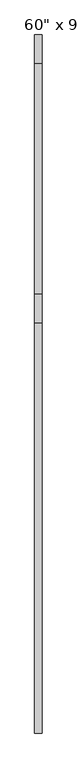
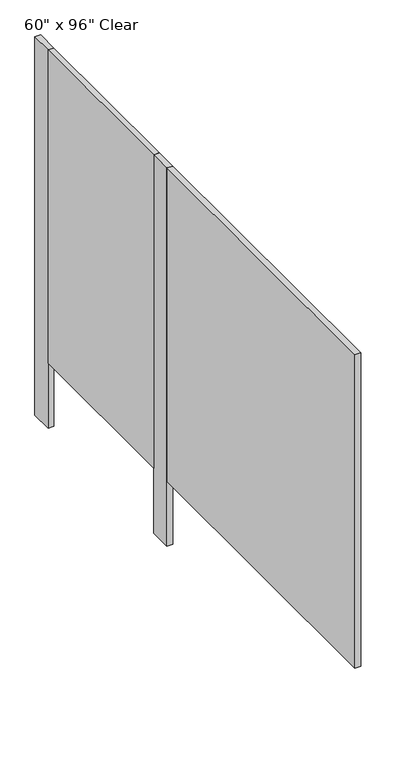
"""IFC4 building model written with IfcOpenShell, lengths in millimetres: proxy geometry."""

import ifcopenshell
import ifcopenshell.guid

model = None  # the IFC model being written
_history = None  # IfcOwnerHistory: only IFC2X3 demands one
_inside = {}  # id of a spatial element -> (the spatial element, [elements in it])
_under = {}  # id of a project, library or spatial element -> (it, [spatial elements below it])
_declared = {}  # id of a project -> (the project, [libraries it declares])
_typed = {}  # id of a type object -> (the type object, [elements of that type])
_made_of = {}  # id of a material, layer set ... -> (it, [elements and type objects made of it])


def new_model(schema):
    """Start an empty IFC model of exactly this schema.

    Asked for "IFC4X3", IfcOpenShell would pick the latest addendum, in which some entities
    have other attributes; the version numbers below select the first issue.
    IFC2X3 requires an IfcOwnerHistory on every rooted entity: one is made here for all.
    """
    global model, _history
    if schema == "IFC4X3":
        model = ifcopenshell.file(schema_version=(4, 3, 0, 0))
    else:
        model = ifcopenshell.file(schema=schema)
    _inside.clear()
    _under.clear()
    _declared.clear()
    _typed.clear()
    _made_of.clear()
    _history = None
    if model.schema == "IFC2X3":
        org = make("IfcOrganization", Name="unknown")
        user = make(
            "IfcPersonAndOrganization",
            ThePerson=make("IfcPerson", FamilyName="unknown"),
            TheOrganization=org,
        )
        app = make(
            "IfcApplication",
            ApplicationDeveloper=org,
            Version="unknown",
            ApplicationFullName="unknown",
            ApplicationIdentifier="unknown",
        )
        _history = make(
            "IfcOwnerHistory",
            OwningUser=user,
            OwningApplication=app,
            ChangeAction="ADDED",
            CreationDate=0,
        )
    return model


def make(cls, **values):
    """One entity of the class cls with the attributes given. An attribute that is None is left unset."""
    return model.create_entity(
        cls, **{name: value for name, value in values.items() if value is not None}
    )


def rooted(cls, **values):
    """An entity with a GlobalId (a new one), such as an element, a storey or a relation."""
    return make(cls, GlobalId=ifcopenshell.guid.new(), OwnerHistory=_history, **values)


def si_unit(unit_type, name, prefix=None):
    """IfcSIUnit, for example si_unit("LENGTHUNIT", "METRE", prefix="MILLI")."""
    return make("IfcSIUnit", UnitType=unit_type, Prefix=prefix, Name=name)


def assignment(units):
    """IfcUnitAssignment: the units of a project."""
    return None if units is None else make("IfcUnitAssignment", Units=units)


def point(xyz):
    """IfcCartesianPoint."""
    return None if xyz is None else make("IfcCartesianPoint", Coordinates=xyz)


def direction(xyz):
    """IfcDirection."""
    return None if xyz is None else make("IfcDirection", DirectionRatios=xyz)


def frame(location, z_axis=None, x_axis=None):
    """IfcAxis2Placement3D, a coordinate frame: its origin and axes. An axis left out is left unset."""
    return make(
        "IfcAxis2Placement3D",
        Location=point(location),
        Axis=direction(z_axis),
        RefDirection=direction(x_axis),
    )


def origin():
    """The frame at (0, 0, 0) with its axes left unset."""
    return frame((0.0, 0.0, 0.0))


def origin_with_axes():
    """The frame at (0, 0, 0) with the z axis (0, 0, 1) and the x axis (1, 0, 0) written out."""
    return frame((0.0, 0.0, 0.0), z_axis=(0.0, 0.0, 1.0), x_axis=(1.0, 0.0, 0.0))


def place(relative_to, where):
    """IfcLocalPlacement: puts the frame where relative to a parent placement (None: the world)."""
    return make(
        "IfcLocalPlacement", PlacementRelTo=relative_to, RelativePlacement=where
    )


def context(
    kind, dimensions, precision=None, world=None, true_north=None, identifier=None
):
    """IfcGeometricRepresentationContext, for example the 3D "Model" context."""
    return make(
        "IfcGeometricRepresentationContext",
        ContextIdentifier=identifier,
        ContextType=kind,
        CoordinateSpaceDimension=dimensions,
        Precision=precision,
        WorldCoordinateSystem=world,
        TrueNorth=true_north,
    )


def project(units=None, contexts=None):
    """IfcProject with its units and contexts."""
    return rooted(
        "IfcProject",
        Name="project",
        RepresentationContexts=contexts,
        UnitsInContext=assignment(units),
    )


def spatial(cls, under=None, at=None, **own):
    """A site, building, storey or space (cls), placed at a placement, below another one or the project."""
    s = rooted(cls, ObjectPlacement=at, **own)
    if under is not None:
        _under.setdefault(under.id(), (under, []))[1].append(s)
    return s


def polyline(points):
    """IfcPolyline through the points."""
    return make("IfcPolyline", Points=[point(p) for p in points])


def outline(outer, holes=None, kind="AREA"):
    """IfcArbitraryClosedProfileDef: a profile drawn as a closed curve; with holes, ...WithVoids."""
    if holes is None:
        return make("IfcArbitraryClosedProfileDef", ProfileType=kind, OuterCurve=outer)
    return make(
        "IfcArbitraryProfileDefWithVoids",
        ProfileType=kind,
        OuterCurve=outer,
        InnerCurves=holes,
    )


def extrude(swept, where, along, depth):
    """IfcExtrudedAreaSolid: the profile swept, set in the frame where, extruded along a direction by depth."""
    return make(
        "IfcExtrudedAreaSolid",
        SweptArea=swept,
        Position=where,
        ExtrudedDirection=direction(along),
        Depth=depth,
    )


def shape(context_of_items, identifier, shape_type, items):
    """IfcShapeRepresentation: the items that make up one representation, for example the "Body"."""
    return make(
        "IfcShapeRepresentation",
        ContextOfItems=context_of_items,
        RepresentationIdentifier=identifier,
        RepresentationType=shape_type,
        Items=items,
    )


def source(mapping_origin, context_of_items, identifier, shape_type, items):
    """IfcRepresentationMap: a shape defined once, which mapped items show again and again."""
    return make(
        "IfcRepresentationMap",
        MappingOrigin=mapping_origin,
        MappedRepresentation=shape(context_of_items, identifier, shape_type, items),
    )


def transform(
    local_origin,
    x_axis=None,
    y_axis=None,
    z_axis=None,
    scale=None,
    scale2=None,
    scale3=None,
    uniform=True,
):
    """IfcCartesianTransformationOperator3D, or its non-uniform kind. x_axis, y_axis, z_axis: its Axis1, 2, 3."""
    if uniform:
        return make(
            "IfcCartesianTransformationOperator3D",
            Axis1=direction(x_axis),
            Axis2=direction(y_axis),
            LocalOrigin=point(local_origin),
            Scale=scale,
            Axis3=direction(z_axis),
        )
    return make(
        "IfcCartesianTransformationOperator3DnonUniform",
        Axis1=direction(x_axis),
        Axis2=direction(y_axis),
        LocalOrigin=point(local_origin),
        Scale=scale,
        Axis3=direction(z_axis),
        Scale2=scale2,
        Scale3=scale3,
    )


def mapped(mapping_source, mapping_target):
    """IfcMappedItem: shows the shape of a source again, moved by a transform."""
    return make(
        "IfcMappedItem", MappingSource=mapping_source, MappingTarget=mapping_target
    )


def made_of(thing, what):
    """Note that an element or type object is made of a material, layer set ...; save() writes the relation."""
    if what is not None:
        _made_of.setdefault(what.id(), (what, []))[1].append(thing)
    return thing


def element(
    cls,
    number,
    at=None,
    inside=None,
    cuts=None,
    type_object=None,
    material=None,
    context=None,
    identifier="Body",
    shape_type=None,
    held_by="IfcProductDefinitionShape",
    body=None,
    shapes=None,
    **own,
):
    """One element of the class cls, such as IfcWall. Its Tag is "e" and its number.

    at: its placement. inside: the storey or other place that contains it. cuts: it is an
    opening in that element (IfcRelVoidsElement). A single representation is given by context,
    identifier, shape_type and body (its items); several are given by shapes. held_by: the class
    of the entity that holds the representations. save() writes the other relations.
    """
    e = rooted(cls, Tag="e%d" % number, ObjectPlacement=at, **own)
    if body is not None:
        shapes = [shape(context, identifier, shape_type, body)]
    if shapes is not None:
        e.Representation = make(held_by, Representations=shapes)
    if inside is not None:
        _inside.setdefault(inside.id(), (inside, []))[1].append(e)
    if cuts is not None:
        rooted(
            "IfcRelVoidsElement", RelatingBuildingElement=cuts, RelatedOpeningElement=e
        )
    if type_object is not None:
        _typed.setdefault(type_object.id(), (type_object, []))[1].append(e)
    return made_of(e, material)


def aggregate(whole, parts):
    """IfcRelAggregates: a whole, such as a stair, and the parts it consists of."""
    return rooted("IfcRelAggregates", RelatingObject=whole, RelatedObjects=parts)


def save(model, path):
    """Write the relations noted so far, then the file.

    IfcRelAggregates (storeys below a building ...), IfcRelContainedInSpatialStructure (elements
    in a storey), IfcRelDefinesByType, IfcRelAssociatesMaterial and IfcRelDeclares: one each for
    every whole, place, type object, material and project.
    """
    for whole, parts in _under.values():
        aggregate(whole, parts)
    for where, things in _inside.values():
        rooted(
            "IfcRelContainedInSpatialStructure",
            RelatedElements=things,
            RelatingStructure=where,
        )
    for kind, things in _typed.values():
        rooted("IfcRelDefinesByType", RelatedObjects=things, RelatingType=kind)
    for what, things in _made_of.values():
        rooted("IfcRelAssociatesMaterial", RelatedObjects=things, RelatingMaterial=what)
    for by, libraries in _declared.values():
        rooted("IfcRelDeclares", RelatingContext=by, RelatedDefinitions=libraries)
    model.write(path)


def proxy_d530cf2d(model_context):
    return source(origin(), model_context, "Body", "SweptSolid", [
        extrude(outline(polyline([(-661.8968462, 2560.6375), (-661.8968462, 1747.8375), (-687.2968462, 1747.8375), (-687.2968462, 2560.6375), (-661.8968462, 2560.6375)])), frame((0.0, 0.0, 304.8), z_axis=(0.0, 0.0, 1.0), x_axis=(1.0, 0.0, 0.0)), (0.0, 0.0, 1.0), 1473.2),
        extrude(outline(polyline([(-661.8968462, 2662.2375), (-661.8968462, 2560.6375), (-687.2968462, 2560.6375), (-687.2968462, 2662.2375), (-661.8968462, 2662.2375)])), origin_with_axes(), (0.0, 0.0, 1.0), 1778.0),
        extrude(outline(polyline([(-661.8968462, 1747.8375), (-661.8968462, 1646.2375), (-687.2968462, 1646.2375), (-687.2968462, 1747.8375), (-661.8968462, 1747.8375)])), origin_with_axes(), (0.0, 0.0, 1.0), 1778.0),
        extrude(outline(polyline([(-687.2968462, 1646.2375), (-661.8968462, 1646.2375), (-661.8968462, 198.4375), (-687.2968462, 198.4375), (-687.2968462, 1646.2375)])), frame((0.0, 0.0, 304.8), z_axis=(0.0, 0.0, 1.0), x_axis=(1.0, 0.0, 0.0)), (0.0, 0.0, 1.0), 1473.2),
    ])


if __name__ == "__main__":
    model = new_model("IFC4")
    model_context = context("Model", 3, world=origin())
    ifc_project = project(units=[si_unit("LENGTHUNIT", "METRE", prefix="MILLI")], contexts=[model_context])
    site = spatial("IfcSite", under=ifc_project)
    building = spatial("IfcBuilding", under=site)
    placement = place(None, origin())
    proxy_shape = proxy_d530cf2d(model_context)
    element("IfcBuildingElementProxy", 1, Name="Toilet Stall-Accessible-Side-3D w Toilet : 60\" x 96\" Clear", ObjectType="Toilet Stall-Accessible-Side-3D w Toilet : 60\" x 96\" Clear", at=placement, inside=building, context=model_context, shape_type="MappedRepresentation", body=[
        mapped(proxy_shape, transform((0.0, 0.0, 0.0), x_axis=(1.0, 0.0, 0.0), y_axis=(0.0, 1.0, 0.0), z_axis=(0.0, 0.0, 1.0))),
    ])
    save(model, "model.ifc")

# Revit data of these elements
# Type "Toilet Stall-Accessible-Side-3D w Toilet : 60\" x 96\" Clear"
#   Assembly Code = "C1030100"
#   Door Width = 2' - 8"
#   Length = 8' - 0"
#   Width = 5' - 0"
#   Show End Panel [instance default] = yes
#   Toilet Partition Material = Toilet Partition
#   Default Elevation = 0
# Element 1 (IfcBuildingElementProxy, "Toilet Stall-Accessible-Side-3D w Toilet : 60\" x 96\" Clear")
#   Show End Panel = no
#   Materials on its faces: "Toilet Partition"
# Materials
#   "Toilet Partition": class "Unassigned", colour RGB 0 181 188, transparency 0
